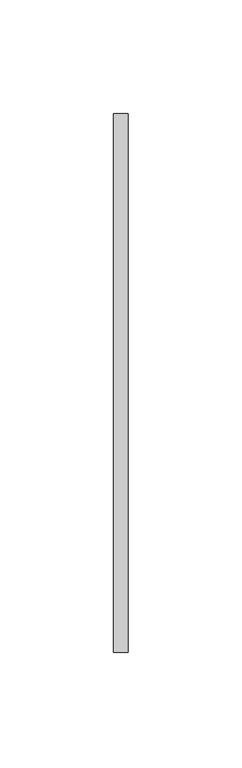
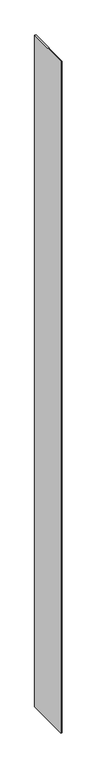
"""IFC4 building model written with IfcOpenShell, lengths in millimetres: proxy geometry, Inner panel1:Inner panel:306176:Inner panel:306176 : Inner panel1:Inner panel:306176:300391:Inner panel:306176:Inner panel:306176 : Inner panel1:Inner panel:306176:300391 : Inner panel1:Inner panel:306176:Inner panel:306176 : Inner panel1:Inner panel:306176:300391:4 : Inner panel1:Inner panel:306176:Inner panel:306176 : Inner panel1:Inner panel:306176:300391:Inner panel:306176:Inner panel:306176 : Inner panel1:Inner panel:306176:300391 : Inner panel1:Inner panel:306176:Inner panel:306176 : Inner panel1:Inner panel:306176:300391:300168."""

from ifc_helpers import new_model, si_unit, frame, origin, place, context, project, spatial, polyline, outline, extrude, source, transform, mapped, element, save


def generic_models_f2a210ff(model_context):
    return source(origin(), model_context, "Body", "SweptSolid", [
        extrude(outline(polyline([(596203.4742239, -579014.9788841), (596203.4742239, -578778.4413841), (596209.8242239, -578778.4413841), (596209.8242239, -579014.9788841), (596203.4742239, -579014.9788841)])), frame((0.0, 0.0, 25.4), z_axis=(0.0, 0.0, 1.0), x_axis=(1.0, 0.0, 0.0)), (0.0, 0.0, 1.0), 3689.35),
    ])


if __name__ == "__main__":
    model = new_model("IFC4")
    model_context = context("Model", 3, world=origin())
    ifc_project = project(units=[si_unit("LENGTHUNIT", "METRE", prefix="MILLI")], contexts=[model_context])
    site = spatial("IfcSite", under=ifc_project)
    building = spatial("IfcBuilding", under=site)
    placement = place(None, origin())
    generic_models_shape = generic_models_f2a210ff(model_context)
    element("IfcBuildingElementProxy", 1, Name="Inner panel1:Inner panel:306176:Inner panel:306176 : Inner panel1:Inner panel:306176:300391:Inner panel:306176:Inner panel:306176 : Inner panel1:Inner panel:306176:300391 : Inner panel1:Inner panel:306176:Inner panel:306176 : Inner panel1:Inner panel:306176:300391:4 : Inner panel1:Inner panel:306176:Inner panel:306176 : Inner panel1:Inner panel:306176:300391:Inner panel:306176:Inner panel:306176 : Inner panel1:Inner panel:306176:300391 : Inner panel1:Inner panel:306176:Inner panel:306176 : Inner panel1:Inner panel:306176:300391:300168", ObjectType="Inner panel1:Inner panel:306176:Inner panel:306176 : Inner panel1:Inner panel:306176:300391:Inner panel:306176:Inner panel:306176 : Inner panel1:Inner panel:306176:300391 : Inner panel1:Inner panel:306176:Inner panel:306176 : Inner panel1:Inner panel:306176:300391:4 : Inner panel1:Inner panel:306176:Inner panel:306176 : Inner panel1:Inner panel:306176:300391:Inner panel:306176:Inner panel:306176 : Inner panel1:Inner panel:306176:300391 : Inner panel1:Inner panel:306176:Inner panel:306176 : Inner panel1:Inner panel:306176:300391:300168", at=placement, inside=building, context=model_context, shape_type="MappedRepresentation", body=[
        mapped(generic_models_shape, transform((0.0, 0.0, 0.0), x_axis=(1.0, 0.0, 0.0), y_axis=(0.0, 1.0, 0.0), z_axis=(0.0, 0.0, 1.0))),
    ])
    save(model, "model.ifc")

# Revit data of these elements
# Type "Inner panel1:Inner panel:306176:Inner panel:306176 : Inner panel1:Inner panel:306176:300391:Inner panel:306176:Inner panel:306176 : Inner panel1:Inner panel:306176:300391 : Inner panel1:Inner panel:306176:Inner panel:306176 : Inner panel1:Inner panel:306176:300391:4 : Inner panel1:Inner panel:306176:Inner panel:306176 : Inner panel1:Inner panel:306176:300391:Inner panel:306176:Inner panel:306176 : Inner panel1:Inner panel:306176:300391 : Inner panel1:Inner panel:306176:Inner panel:306176 : Inner panel1:Inner panel:306176:300391:300168"
#   NameOverride = "Inner panel1:Inner panel:306176:Inner panel:306176 : Inner panel1:Inner panel:306176:300391:Inner panel:306176:Inner panel:306176 : Inner panel1:Inner panel:306176:300391 : Inner panel1:Inner panel:306176:Inner panel:306176 : Inner panel1:Inner panel:306176:300391:300168"
#   ObjectTypeOverride = "Inner panel:306176:Inner panel:306176 : Inner panel1:Inner panel:306176:300391 : Inner panel1:Inner panel:306176:Inner panel:306176 : Inner panel1:Inner panel:306176:300391"
#   Reference = "Inner panel"
#   Tag = "300168"
# Element 1 (IfcBuildingElementProxy, "Inner panel1:Inner panel:306176:Inner panel:306176 : Inner panel1:Inner panel:306176:300391:Inner panel:306176:Inner panel:306176 : Inner panel1:Inner panel:306176:300391 : Inner panel1:Inner panel:306176:Inner panel:306176 : Inner panel1:Inner panel:306176:300391:4 : Inner panel1:Inner panel:306176:Inner panel:306176 : Inner panel1:Inner panel:306176:300391:Inner panel:306176:Inner panel:306176 : Inner panel1:Inner panel:306176:300391 : Inner panel1:Inner panel:306176:Inner panel:306176 : Inner panel1:Inner panel:306176:300391:300168")
#   Materials on its faces: "1/4\" CEMENT BOARD"
# Materials
#   "1/4\" CEMENT BOARD": class "Generic", colour RGB 234 234 234, transparency 0, Cost = 0
